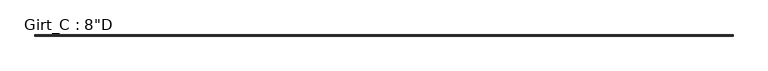
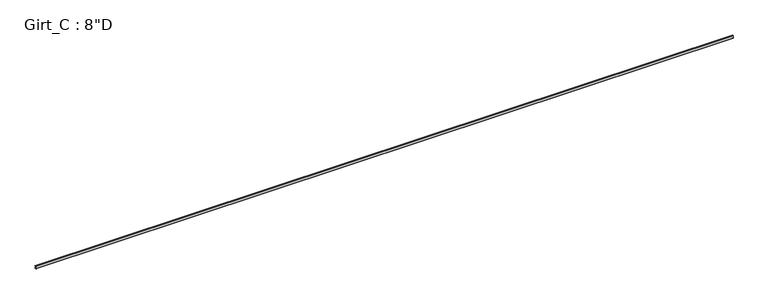
"""IFC4 building model written with IfcOpenShell, lengths in millimetres: beam geometry."""

import ifcopenshell
import ifcopenshell.guid

model = None  # the IFC model being written
_history = None  # IfcOwnerHistory: only IFC2X3 demands one
_inside = {}  # id of a spatial element -> (the spatial element, [elements in it])
_under = {}  # id of a project, library or spatial element -> (it, [spatial elements below it])
_declared = {}  # id of a project -> (the project, [libraries it declares])
_typed = {}  # id of a type object -> (the type object, [elements of that type])
_made_of = {}  # id of a material, layer set ... -> (it, [elements and type objects made of it])


def new_model(schema):
    """Start an empty IFC model of exactly this schema.

    Asked for "IFC4X3", IfcOpenShell would pick the latest addendum, in which some entities
    have other attributes; the version numbers below select the first issue.
    IFC2X3 requires an IfcOwnerHistory on every rooted entity: one is made here for all.
    """
    global model, _history
    if schema == "IFC4X3":
        model = ifcopenshell.file(schema_version=(4, 3, 0, 0))
    else:
        model = ifcopenshell.file(schema=schema)
    _inside.clear()
    _under.clear()
    _declared.clear()
    _typed.clear()
    _made_of.clear()
    _history = None
    if model.schema == "IFC2X3":
        org = make("IfcOrganization", Name="unknown")
        user = make(
            "IfcPersonAndOrganization",
            ThePerson=make("IfcPerson", FamilyName="unknown"),
            TheOrganization=org,
        )
        app = make(
            "IfcApplication",
            ApplicationDeveloper=org,
            Version="unknown",
            ApplicationFullName="unknown",
            ApplicationIdentifier="unknown",
        )
        _history = make(
            "IfcOwnerHistory",
            OwningUser=user,
            OwningApplication=app,
            ChangeAction="ADDED",
            CreationDate=0,
        )
    return model


def make(cls, **values):
    """One entity of the class cls with the attributes given. An attribute that is None is left unset."""
    return model.create_entity(
        cls, **{name: value for name, value in values.items() if value is not None}
    )


def rooted(cls, **values):
    """An entity with a GlobalId (a new one), such as an element, a storey or a relation."""
    return make(cls, GlobalId=ifcopenshell.guid.new(), OwnerHistory=_history, **values)


def si_unit(unit_type, name, prefix=None):
    """IfcSIUnit, for example si_unit("LENGTHUNIT", "METRE", prefix="MILLI")."""
    return make("IfcSIUnit", UnitType=unit_type, Prefix=prefix, Name=name)


def assignment(units):
    """IfcUnitAssignment: the units of a project."""
    return None if units is None else make("IfcUnitAssignment", Units=units)


def point(xyz):
    """IfcCartesianPoint."""
    return None if xyz is None else make("IfcCartesianPoint", Coordinates=xyz)


def direction(xyz):
    """IfcDirection."""
    return None if xyz is None else make("IfcDirection", DirectionRatios=xyz)


def frame(location, z_axis=None, x_axis=None):
    """IfcAxis2Placement3D, a coordinate frame: its origin and axes. An axis left out is left unset."""
    return make(
        "IfcAxis2Placement3D",
        Location=point(location),
        Axis=direction(z_axis),
        RefDirection=direction(x_axis),
    )


def frame_2d(location, x_axis=None):
    """IfcAxis2Placement2D, a coordinate frame in the plane: its origin and x axis."""
    return make(
        "IfcAxis2Placement2D", Location=point(location), RefDirection=direction(x_axis)
    )


def origin():
    """The frame at (0, 0, 0) with its axes left unset."""
    return frame((0.0, 0.0, 0.0))


def place(relative_to, where):
    """IfcLocalPlacement: puts the frame where relative to a parent placement (None: the world)."""
    return make(
        "IfcLocalPlacement", PlacementRelTo=relative_to, RelativePlacement=where
    )


def context(
    kind, dimensions, precision=None, world=None, true_north=None, identifier=None
):
    """IfcGeometricRepresentationContext, for example the 3D "Model" context."""
    return make(
        "IfcGeometricRepresentationContext",
        ContextIdentifier=identifier,
        ContextType=kind,
        CoordinateSpaceDimension=dimensions,
        Precision=precision,
        WorldCoordinateSystem=world,
        TrueNorth=true_north,
    )


def project(units=None, contexts=None):
    """IfcProject with its units and contexts."""
    return rooted(
        "IfcProject",
        Name="project",
        RepresentationContexts=contexts,
        UnitsInContext=assignment(units),
    )


def spatial(cls, under=None, at=None, **own):
    """A site, building, storey or space (cls), placed at a placement, below another one or the project."""
    s = rooted(cls, ObjectPlacement=at, **own)
    if under is not None:
        _under.setdefault(under.id(), (under, []))[1].append(s)
    return s


def polyline(points):
    """IfcPolyline through the points."""
    return make("IfcPolyline", Points=[point(p) for p in points])


def circle_curve(where, radius):
    """IfcCircle in the frame where."""
    return make("IfcCircle", Position=where, Radius=radius)


def trimmed(basis, trim1, trim2, sense, master):
    """IfcTrimmedCurve: the piece of a basis curve between two trims."""
    return make(
        "IfcTrimmedCurve",
        BasisCurve=basis,
        Trim1=trim1,
        Trim2=trim2,
        SenseAgreement=sense,
        MasterRepresentation=master,
    )


def segment(curve, same_sense, transition):
    """IfcCompositeCurveSegment."""
    return make(
        "IfcCompositeCurveSegment",
        Transition=transition,
        SameSense=same_sense,
        ParentCurve=curve,
    )


def composite_curve(segments, self_intersect=None):
    """IfcCompositeCurve: segments joined end to end."""
    return make("IfcCompositeCurve", Segments=segments, SelfIntersect=self_intersect)


def outline(outer, holes=None, kind="AREA"):
    """IfcArbitraryClosedProfileDef: a profile drawn as a closed curve; with holes, ...WithVoids."""
    if holes is None:
        return make("IfcArbitraryClosedProfileDef", ProfileType=kind, OuterCurve=outer)
    return make(
        "IfcArbitraryProfileDefWithVoids",
        ProfileType=kind,
        OuterCurve=outer,
        InnerCurves=holes,
    )


def extrude(swept, where, along, depth):
    """IfcExtrudedAreaSolid: the profile swept, set in the frame where, extruded along a direction by depth."""
    return make(
        "IfcExtrudedAreaSolid",
        SweptArea=swept,
        Position=where,
        ExtrudedDirection=direction(along),
        Depth=depth,
    )


def shape(context_of_items, identifier, shape_type, items):
    """IfcShapeRepresentation: the items that make up one representation, for example the "Body"."""
    return make(
        "IfcShapeRepresentation",
        ContextOfItems=context_of_items,
        RepresentationIdentifier=identifier,
        RepresentationType=shape_type,
        Items=items,
    )


def source(mapping_origin, context_of_items, identifier, shape_type, items):
    """IfcRepresentationMap: a shape defined once, which mapped items show again and again."""
    return make(
        "IfcRepresentationMap",
        MappingOrigin=mapping_origin,
        MappedRepresentation=shape(context_of_items, identifier, shape_type, items),
    )


def transform(
    local_origin,
    x_axis=None,
    y_axis=None,
    z_axis=None,
    scale=None,
    scale2=None,
    scale3=None,
    uniform=True,
):
    """IfcCartesianTransformationOperator3D, or its non-uniform kind. x_axis, y_axis, z_axis: its Axis1, 2, 3."""
    if uniform:
        return make(
            "IfcCartesianTransformationOperator3D",
            Axis1=direction(x_axis),
            Axis2=direction(y_axis),
            LocalOrigin=point(local_origin),
            Scale=scale,
            Axis3=direction(z_axis),
        )
    return make(
        "IfcCartesianTransformationOperator3DnonUniform",
        Axis1=direction(x_axis),
        Axis2=direction(y_axis),
        LocalOrigin=point(local_origin),
        Scale=scale,
        Axis3=direction(z_axis),
        Scale2=scale2,
        Scale3=scale3,
    )


def mapped(mapping_source, mapping_target):
    """IfcMappedItem: shows the shape of a source again, moved by a transform."""
    return make(
        "IfcMappedItem", MappingSource=mapping_source, MappingTarget=mapping_target
    )


def made_of(thing, what):
    """Note that an element or type object is made of a material, layer set ...; save() writes the relation."""
    if what is not None:
        _made_of.setdefault(what.id(), (what, []))[1].append(thing)
    return thing


def element(
    cls,
    number,
    at=None,
    inside=None,
    cuts=None,
    type_object=None,
    material=None,
    context=None,
    identifier="Body",
    shape_type=None,
    held_by="IfcProductDefinitionShape",
    body=None,
    shapes=None,
    **own,
):
    """One element of the class cls, such as IfcWall. Its Tag is "e" and its number.

    at: its placement. inside: the storey or other place that contains it. cuts: it is an
    opening in that element (IfcRelVoidsElement). A single representation is given by context,
    identifier, shape_type and body (its items); several are given by shapes. held_by: the class
    of the entity that holds the representations. save() writes the other relations.
    """
    e = rooted(cls, Tag="e%d" % number, ObjectPlacement=at, **own)
    if body is not None:
        shapes = [shape(context, identifier, shape_type, body)]
    if shapes is not None:
        e.Representation = make(held_by, Representations=shapes)
    if inside is not None:
        _inside.setdefault(inside.id(), (inside, []))[1].append(e)
    if cuts is not None:
        rooted(
            "IfcRelVoidsElement", RelatingBuildingElement=cuts, RelatedOpeningElement=e
        )
    if type_object is not None:
        _typed.setdefault(type_object.id(), (type_object, []))[1].append(e)
    return made_of(e, material)


def aggregate(whole, parts):
    """IfcRelAggregates: a whole, such as a stair, and the parts it consists of."""
    return rooted("IfcRelAggregates", RelatingObject=whole, RelatedObjects=parts)


def save(model, path):
    """Write the relations noted so far, then the file.

    IfcRelAggregates (storeys below a building ...), IfcRelContainedInSpatialStructure (elements
    in a storey), IfcRelDefinesByType, IfcRelAssociatesMaterial and IfcRelDeclares: one each for
    every whole, place, type object, material and project.
    """
    for whole, parts in _under.values():
        aggregate(whole, parts)
    for where, things in _inside.values():
        rooted(
            "IfcRelContainedInSpatialStructure",
            RelatedElements=things,
            RelatingStructure=where,
        )
    for kind, things in _typed.values():
        rooted("IfcRelDefinesByType", RelatedObjects=things, RelatingType=kind)
    for what, things in _made_of.values():
        rooted("IfcRelAssociatesMaterial", RelatedObjects=things, RelatingMaterial=what)
    for by, libraries in _declared.values():
        rooted("IfcRelDeclares", RelatingContext=by, RelatedDefinitions=libraries)
    model.write(path)


def beam_fa770e31(model_context):
    return source(origin(), model_context, "Body", "SweptSolid", [
        extrude(outline(composite_curve([segment(polyline([(63.5, 101.6), (75.745104, 87.0068534), (73.6169367, 85.221109), (62.204539, 98.821875), (3.3005807, 98.821875)]), True, "CONTINUOUS"), segment(trimmed(circle_curve(frame_2d((3.3741066, 96.8381931)), 1.9850441), [point((3.3005807, 98.821875))], [point((1.3890625, 96.8381931))], True, "CARTESIAN"), True, "CONTINUOUS"), segment(polyline([(1.3890625, 96.8381931), (1.3890625, -96.8389339)]), True, "CONTINUOUS"), segment(trimmed(circle_curve(frame_2d((3.3748024, -96.8389339)), 1.9857399), [point((1.3890625, -96.8389339))], [point((3.2694106, -98.821875))], True, "CARTESIAN"), True, "CONTINUOUS"), segment(polyline([(3.2694106, -98.821875), (62.204539, -98.821875), (73.6169367, -85.221109), (75.745104, -87.0068534), (63.5, -101.6), (3.3734375, -101.6)]), True, "CONTINUOUS"), segment(trimmed(circle_curve(frame_2d((3.3734375, -96.8375)), 4.7625), [point((3.3734375, -101.6))], [point((-1.3890625, -96.8375))], False, "CARTESIAN"), True, "CONTINUOUS"), segment(polyline([(-1.3890625, -96.8375), (-1.3890625, 96.8375)]), True, "CONTINUOUS"), segment(trimmed(circle_curve(frame_2d((3.3734375, 96.8375)), 4.7625), [point((-1.3890625, 96.8375))], [point((3.3734375, 101.6))], False, "CARTESIAN"), True, "CONTINUOUS"), segment(polyline([(3.3734375, 101.6), (63.5, 101.6)]), True, "CONTINUOUS")], self_intersect=False)), frame((-24463.375, 0.0, 0.0), z_axis=(1.0, 0.0, 0.0), x_axis=(0.0, 1.0, 0.0)), (0.0, 0.0, 1.0), 48926.75),
    ])


if __name__ == "__main__":
    model = new_model("IFC4")
    model_context = context("Model", 3, world=origin())
    ifc_project = project(units=[si_unit("LENGTHUNIT", "METRE", prefix="MILLI")], contexts=[model_context])
    site = spatial("IfcSite", under=ifc_project)
    building = spatial("IfcBuilding", under=site)
    placement = place(None, origin())
    beam_shape = beam_fa770e31(model_context)
    element("IfcBeam", 1, ObjectType="Girt_C : 8\"D", at=placement, inside=building, context=model_context, shape_type="MappedRepresentation", body=[
        mapped(beam_shape, transform((0.0, 0.0, 0.0), x_axis=(1.0, 0.0, 0.0), y_axis=(0.0, 1.0, 0.0), z_axis=(0.0, 0.0, 1.0))),
    ])
    save(model, "model.ifc")

# Revit data of these elements
# Type "Girt_C : 8\"D"
#   Web_Thickness = 0' - 0 7/64"
#   Length [instance default] = 10' - 0"
#   Leg_1 = 0' - 2 1/2"
#   Height = 0' - 8"
#   Structural Material [instance default] = none
# Element 1 (IfcBeam, "Girt_C : 8\"D")
#   Materials on its faces: "Steel"
# Materials
#   "Steel": class "Metal", colour RGB 118 118 114, transparency 0, Description = "Steel, mill finish", Cost = 0
